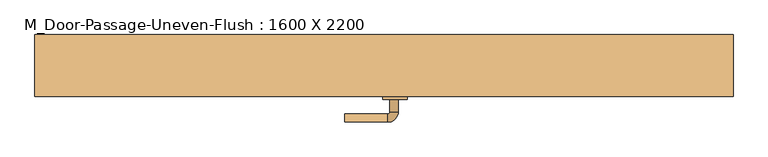
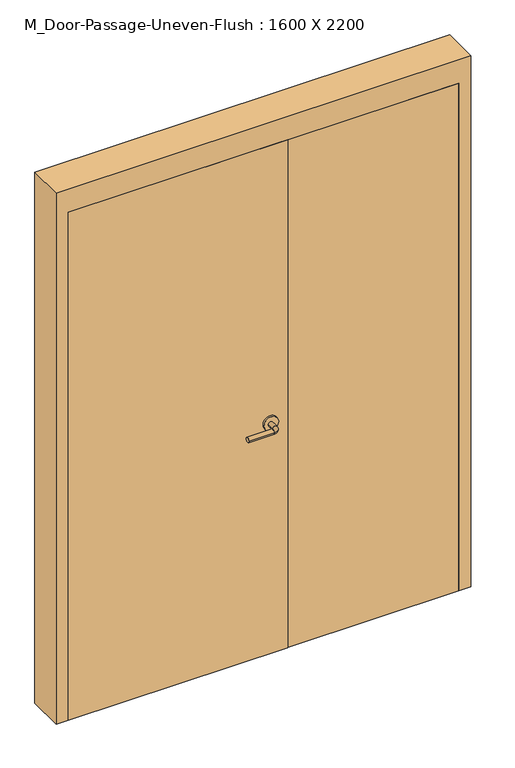
"""IFC4 building model written with IfcOpenShell, lengths in millimetres: door geometry, M_Door-Passage-Uneven-Flush : 1600 X 2200."""

from ifc_helpers import new_model, si_unit, point, frame, frame_2d, origin, origin_with_axes, place, context, project, spatial, polyline, circle_curve, ellipse_curve, trimmed, segment, composite_curve, outline, extrude, faceted_brep, source, transform, mapped, element, save
from ifc_brep_helpers import plane_surface, cylinder_surface, revolved_surface, advanced_brep


def m_door_passage_uneven_flush_1600_x_2200_848efb9c(model_context):
    return source(origin(), model_context, "Body", "SolidModel", [
        advanced_brep(
        [(34.59375, 9.15, 1000.0), (14.59375, 9.15, 1000.0), (14.59375, 39.15, 1000.0), (34.59375, 39.15, 1000.0), (9.59375, 44.15, 1000.0), (9.59375, 64.15, 1000.0), (-95.40625, 64.15, 1000.0), (-95.40625, 44.15, 1000.0)],
        [
            (0, 1, circle_curve(frame((24.59375, 9.15, 1000.0), z_axis=(0.0, -1.0, 0.0), x_axis=(-1.0, 0.0, 0.0)), 10.0)),
            (1, 0, circle_curve(frame((24.59375, 9.15, 1000.0), z_axis=(0.0, -1.0, 0.0), x_axis=(-1.0, 0.0, 0.0)), 10.0)),
            (1, 2),
            (2, 3, circle_curve(frame((24.59375, 39.15, 1000.0), z_axis=(0.0, -1.0, 0.0), x_axis=(-1.0, 0.0, 0.0)), 10.0)),
            (3, 0),
            (3, 2, circle_curve(frame((24.59375, 39.15, 1000.0), z_axis=(0.0, -1.0, 0.0), x_axis=(-1.0, 0.0, 0.0)), 10.0)),
            (4, 5, circle_curve(frame((9.59375, 54.15, 1000.0), z_axis=(1.0, 0.0, 0.0), x_axis=(0.0, -1.0, 0.0)), 10.0)),
            (5, 3, circle_curve(frame((9.59375, 39.15, 1000.0), z_axis=(0.0, 0.0, -1.0), x_axis=(1.0, 0.0, 0.0)), 25.0)),
            (2, 4, circle_curve(frame((9.59375, 39.15, 1000.0), z_axis=(0.0, 0.0, 1.0), x_axis=(1.0, 0.0, 0.0)), 5.0)),
            (5, 4, circle_curve(frame((9.59375, 54.15, 1000.0), z_axis=(1.0, 0.0, 0.0), x_axis=(0.0, -1.0, 0.0)), 10.0)),
            (6, 7, circle_curve(frame((-95.40625, 54.15, 1000.0), z_axis=(-1.0, 0.0, 0.0), x_axis=(0.0, -1.0, 0.0)), 10.0)),
            (7, 6, circle_curve(frame((-95.40625, 54.15, 1000.0), z_axis=(-1.0, 0.0, 0.0), x_axis=(0.0, -1.0, 0.0)), 10.0)),
            (4, 7),
            (6, 5),
        ],
        [
            plane_surface(frame((24.59375, 9.15, 1000.0), z_axis=(0.0, -1.0, 0.0), x_axis=(0.0, 0.0, 1.0))),
            cylinder_surface(frame((24.59375, 9.15, 1000.0), z_axis=(0.0, -1.0, 0.0), x_axis=(-1.0, 0.0, 0.0)), 10.0),
            revolved_surface(trimmed(ellipse_curve(frame((24.59375, 39.15, 1000.0), z_axis=(0.0, 1.0, 0.0), x_axis=(-1.0, 0.0, 0.0)), 10.0, 10.0), [point((34.59375, 39.15, 1000.0))], [point((14.59375, 39.15, 1000.0))], True, "CARTESIAN"), (9.59375, 39.15, 1000.0), (0.0, 0.0, -1.0)),
            revolved_surface(trimmed(ellipse_curve(frame((24.59375, 39.15, 1000.0), z_axis=(0.0, 1.0, 0.0), x_axis=(-1.0, 0.0, 0.0)), 10.0, 10.0), [point((14.59375, 39.15, 1000.0))], [point((34.59375, 39.15, 1000.0))], True, "CARTESIAN"), (9.59375, 39.15, 1000.0), (0.0, 0.0, -1.0)),
            plane_surface(frame((-95.40625, 54.15, 1000.0), z_axis=(-1.0, 0.0, 0.0), x_axis=(0.0, 0.0, 1.0))),
            cylinder_surface(frame((9.59375, 54.15, 1000.0), z_axis=(1.0, 0.0, 0.0), x_axis=(0.0, -1.0, 0.0)), 10.0),
        ],
        [
            (0, [[1, 2]]),
            (1, [[3, 4, 5, -2]]),
            (1, [[-5, 6, -3, -1]]),
            (2, [[7, 8, -4, 9]]),
            (3, [[10, -9, -6, -8]]),
            (4, [[11, 12]]),
            (5, [[13, -11, 14, -7]]),
            (5, [[-14, -12, -13, -10]]),
        ],
    ),
        extrude(outline(composite_curve([segment(trimmed(circle_curve(frame_2d((1000.0, 27.09375)), 30.0), [point((1000.0, 57.09375))], [point((1000.0, -2.90625))], False, "CARTESIAN"), True, "CONTINUOUS"), segment(trimmed(circle_curve(frame_2d((1000.0, 27.09375)), 30.0), [point((1000.0, -2.90625))], [point((1000.0, 57.09375))], False, "CARTESIAN"), True, "CONTINUOUS")], self_intersect=False)), frame((0.0, 1.15, 0.0), z_axis=(0.0, 1.0, 0.0), x_axis=(0.0, 0.0, 1.0)), (0.0, 0.0, 1.0), 8.0),
        advanced_brep(
        [(34.59375, -51.85, 1000.0), (14.59375, -51.85, 1000.0), (34.59375, -81.85, 1000.0), (14.59375, -81.85, 1000.0), (9.59375, -86.85, 1000.0), (9.59375, -106.85, 1000.0), (-95.40625, -106.85, 1000.0), (-95.40625, -86.85, 1000.0)],
        [
            (0, 1, circle_curve(frame((24.59375, -51.85, 1000.0), z_axis=(0.0, 1.0, 0.0), x_axis=(-1.0, 0.0, 0.0)), 10.0)),
            (1, 0, circle_curve(frame((24.59375, -51.85, 1000.0), z_axis=(0.0, 1.0, 0.0), x_axis=(-1.0, 0.0, 0.0)), 10.0)),
            (0, 2),
            (2, 3, circle_curve(frame((24.59375, -81.85, 1000.0), z_axis=(0.0, 1.0, 0.0), x_axis=(-1.0, 0.0, 0.0)), 10.0)),
            (3, 1),
            (3, 2, circle_curve(frame((24.59375, -81.85, 1000.0), z_axis=(0.0, 1.0, 0.0), x_axis=(-1.0, 0.0, 0.0)), 10.0)),
            (4, 3, circle_curve(frame((9.59375, -81.85, 1000.0), z_axis=(0.0, 0.0, 1.0), x_axis=(1.0, 0.0, 0.0)), 5.0)),
            (2, 5, circle_curve(frame((9.59375, -81.85, 1000.0), z_axis=(0.0, 0.0, -1.0), x_axis=(1.0, 0.0, 0.0)), 25.0)),
            (5, 4, circle_curve(frame((9.59375, -96.85, 1000.0), z_axis=(1.0, 0.0, 0.0), x_axis=(0.0, 1.0, 0.0)), 10.0)),
            (4, 5, circle_curve(frame((9.59375, -96.85, 1000.0), z_axis=(1.0, 0.0, 0.0), x_axis=(0.0, 1.0, 0.0)), 10.0)),
            (6, 7, circle_curve(frame((-95.40625, -96.85, 1000.0), z_axis=(-1.0, 0.0, 0.0), x_axis=(0.0, 1.0, 0.0)), 10.0)),
            (7, 6, circle_curve(frame((-95.40625, -96.85, 1000.0), z_axis=(-1.0, 0.0, 0.0), x_axis=(0.0, 1.0, 0.0)), 10.0)),
            (5, 6),
            (7, 4),
        ],
        [
            plane_surface(frame((24.59375, -51.85, 1000.0), z_axis=(0.0, 1.0, 0.0), x_axis=(0.0, 0.0, 1.0))),
            cylinder_surface(frame((24.59375, -51.85, 1000.0), z_axis=(0.0, 1.0, 0.0), x_axis=(-1.0, 0.0, 0.0)), 10.0),
            revolved_surface(trimmed(ellipse_curve(frame((24.59375, -81.85, 1000.0), z_axis=(0.0, 1.0, 0.0), x_axis=(-1.0, 0.0, 0.0)), 10.0, 10.0), [point((34.59375, -81.85, 1000.0))], [point((14.59375, -81.85, 1000.0))], True, "CARTESIAN"), (9.59375, -81.85, 1000.0), (0.0, 0.0, -1.0)),
            revolved_surface(trimmed(ellipse_curve(frame((24.59375, -81.85, 1000.0), z_axis=(0.0, 1.0, 0.0), x_axis=(-1.0, 0.0, 0.0)), 10.0, 10.0), [point((14.59375, -81.85, 1000.0))], [point((34.59375, -81.85, 1000.0))], True, "CARTESIAN"), (9.59375, -81.85, 1000.0), (0.0, 0.0, -1.0)),
            plane_surface(frame((-95.40625, -96.85, 1000.0), z_axis=(-1.0, 0.0, 0.0), x_axis=(0.0, 0.0, 1.0))),
            cylinder_surface(frame((9.59375, -96.85, 1000.0), z_axis=(1.0, 0.0, 0.0), x_axis=(0.0, 1.0, 0.0)), 10.0),
        ],
        [
            (0, [[1, 2]]),
            (1, [[-1, 3, 4, 5]]),
            (1, [[-2, -5, 6, -3]]),
            (2, [[7, -4, 8, 9]]),
            (3, [[-8, -6, -7, 10]]),
            (4, [[11, 12]]),
            (5, [[-9, 13, -12, 14]]),
            (5, [[-10, -14, -11, -13]]),
        ],
    ),
        extrude(outline(composite_curve([segment(trimmed(circle_curve(frame_2d((1000.0, 27.09375)), 30.0), [point((1000.0, 57.09375))], [point((1000.0, -2.90625))], False, "CARTESIAN"), True, "CONTINUOUS"), segment(trimmed(circle_curve(frame_2d((1000.0, 27.09375)), 30.0), [point((1000.0, -2.90625))], [point((1000.0, 57.09375))], False, "CARTESIAN"), True, "CONTINUOUS")], self_intersect=False)), frame((0.0, -51.85, 0.0), z_axis=(0.0, 1.0, 0.0), x_axis=(0.0, 0.0, 1.0)), (0.0, 0.0, 1.0), 8.0),
        extrude(outline(polyline([(98.4, 1.15), (98.4, -43.85), (-800.0, -43.85), (-800.0, 1.15), (98.4, 1.15)])), origin_with_axes(), (0.0, 0.0, 1.0), 2200.0),
        faceted_brep([(800.0, 5.9125, 0.0), (784.125, 5.9125, 0.0), (784.125, 56.9375, 0.0), (800.0, 56.9375, 0.0), (800.0, 106.15, 0.0), (850.0, 106.15, 0.0), (850.0, -43.85, 0.0), (800.0, -43.85, 0.0), (800.0, -43.85, 2200.0), (800.0, 5.9125, 2200.0), (850.0, -43.85, 2300.0), (-850.0, -43.85, 2300.0), (-850.0, -43.85, 0.0), (-800.0, -43.85, 0.0), (-800.0, -43.85, 2200.0), (850.0, 106.15, 2300.0), (800.0, 106.15, 2200.0), (-800.0, 106.15, 2200.0), (-800.0, 106.15, 0.0), (-850.0, 106.15, 0.0), (-850.0, 106.15, 2300.0), (800.0, 56.9375, 2200.0), (784.125, 56.9375, 2184.125), (-784.125, 56.9375, 2184.125), (-784.125, 56.9375, 0.0), (-800.0, 56.9375, 0.0), (-800.0, 56.9375, 2200.0), (784.125, 5.9125, 2184.125), (-800.0, 5.9125, 2200.0), (-800.0, 5.9125, 0.0), (-784.125, 5.9125, 0.0), (-784.125, 5.9125, 2184.125)], [[[0, 1, 2, 3, 4, 5, 6, 7]], [[7, 8, 9, 0]], [[6, 10, 11, 12, 13, 14, 8, 7]], [[5, 15, 10, 6]], [[4, 16, 17, 18, 19, 20, 15, 5]], [[3, 21, 16, 4]], [[2, 22, 23, 24, 25, 26, 21, 3]], [[1, 27, 22, 2]], [[0, 9, 28, 29, 30, 31, 27, 1]], [[8, 14, 28, 9]], [[16, 21, 26, 17]], [[22, 27, 31, 23]], [[12, 19, 18, 25, 24, 30, 29, 13]], [[13, 29, 28, 14]], [[11, 20, 19, 12]], [[17, 26, 25, 18]], [[23, 31, 30, 24]], [[15, 20, 11, 10]]]),
        extrude(outline(polyline([(800.0, 1.15), (800.0, -43.85), (101.6, -43.85), (101.6, 1.15), (800.0, 1.15)])), origin_with_axes(), (0.0, 0.0, 1.0), 2200.0),
    ])


if __name__ == "__main__":
    model = new_model("IFC4")
    model_context = context("Model", 3, world=origin())
    ifc_project = project(units=[si_unit("LENGTHUNIT", "METRE", prefix="MILLI")], contexts=[model_context])
    site = spatial("IfcSite", under=ifc_project)
    building = spatial("IfcBuilding", under=site)
    placement = place(None, origin())
    m_door_passage_uneven_flush_1600_x_2200_shape = m_door_passage_uneven_flush_1600_x_2200_848efb9c(model_context)
    element("IfcDoor", 1, ObjectType="M_Door-Passage-Uneven-Flush : 1600 X 2200", at=placement, inside=building, context=model_context, shape_type="MappedRepresentation", body=[
        mapped(m_door_passage_uneven_flush_1600_x_2200_shape, transform((0.0, 0.0, 0.0), x_axis=(1.0, 0.0, 0.0), y_axis=(0.0, 1.0, 0.0), z_axis=(0.0, 0.0, 1.0))),
    ])
    save(model, "model.ifc")

# Revit data of these elements
# Type "M_Door-Passage-Uneven-Flush : 1600 X 2200"
#   Type Mark = "50"
#   Assembly Code = "C1020300"
#   Analytic Construction = "Wooden"
#   Width Large Panel = 900 mm
#   W = 700 mm
#   Thickness = 45 mm
#   Thermal Resistance (R) = 0.455703 (m²·K)/W
#   Swing Angle [instance default] = 90.00°
#   Strike Height = 1000 mm
#   Rough Width [instance default] = 1700 mm
#   Rough Height [instance default] = 2300 mm
#   Masonry Frame Opening Height [instance default] = 100 mm
#   Masonry Frame Opening Width [instance default] = 100 mm
#   Inset Calculation [instance default] = 105 mm
#   Masonry Inset [instance default] = 25 mm
#   Height = 2200 mm
#   Width = 1600 mm
#   Heat Transfer Coefficient (U) = 2.19465 W/(m²·K)
#   Masonry Frame Depth = 150 mm
#   Masonry Frame [instance default] = yes
#   Dry Wall Frame [instance default] = no
#   Panel Material = Wood - Birch
#   Frame Material = Metal - Paint Finish - Grey
#   Door Handle Material = Aluminum
#   Visual Light Transmittance = 0
#   Solar Heat Gain Coefficient = 0
#   Wall Closure = (empty or 0)
#   Function = (empty or 0)
# Element 1 (IfcDoor, "M_Door-Passage-Uneven-Flush : 1600 X 2200")
#   Materials on its faces: "Aluminum", "Metal - Paint Finish - Grey", "Wood - Birch"
# Materials
#   "Wood - Birch": class "Wood", colour RGB 166 116 52, transparency 0, Cost = 0
#   "Metal - Paint Finish - Grey": class "Paint", colour RGB 104 104 104, transparency 0, Cost = 0
#   "Aluminum": class "Metal", colour RGB 244 244 244, transparency 0, Description = "Aluminum 6061", Cost = 0
